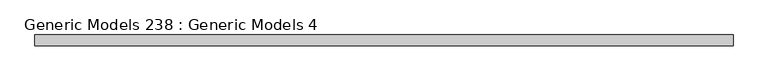
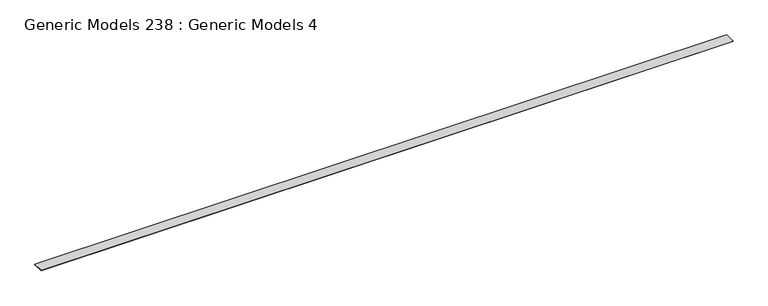
"""IFC4 building model written with IfcOpenShell, lengths in millimetres: proxy geometry, Generic Models 238 : Generic Models 4."""

from ifc_helpers import new_model, si_unit, frame, origin, place, context, project, spatial, polyline, outline, extrude, source, transform, mapped, element, save


def generic_models_238_generic_models_4_992afd31(model_context):
    return source(origin(), model_context, "Body", "SweptSolid", [
        extrude(outline(polyline([(8416.2258303, 11786.2107536), (8416.2258303, 11499.2769662), (-10227.3741697, 11499.2769662), (-10227.3741697, 11786.2107536), (8416.2258303, 11786.2107536)])), frame((0.0, 0.0, 126924.1811183), z_axis=(0.0, 0.0, 1.0), x_axis=(1.0, 0.0, 0.0)), (0.0, 0.0, 1.0), 12.7),
    ])


if __name__ == "__main__":
    model = new_model("IFC4")
    model_context = context("Model", 3, world=origin())
    ifc_project = project(units=[si_unit("LENGTHUNIT", "METRE", prefix="MILLI")], contexts=[model_context])
    site = spatial("IfcSite", under=ifc_project)
    building = spatial("IfcBuilding", under=site)
    placement = place(None, origin())
    generic_models_238_generic_models_4_shape = generic_models_238_generic_models_4_992afd31(model_context)
    element("IfcBuildingElementProxy", 1, Name="Generic Models 238 : Generic Models 4", ObjectType="Generic Models 238 : Generic Models 4", at=placement, inside=building, context=model_context, shape_type="MappedRepresentation", body=[
        mapped(generic_models_238_generic_models_4_shape, transform((0.0, 0.0, 0.0), x_axis=(1.0, 0.0, 0.0), y_axis=(0.0, 1.0, 0.0), z_axis=(0.0, 0.0, 1.0))),
    ])
    save(model, "model.ifc")

# Revit data of these elements
# Element 1 (IfcBuildingElementProxy, "Generic Models 238 : Generic Models 4")
#   Materials on its faces: "_1/2\" CDX PLYWOOD"
# Materials
#   "_1/2\" CDX PLYWOOD": class "Generic", colour RGB 98 75 74, transparency 0, Cost = 0
